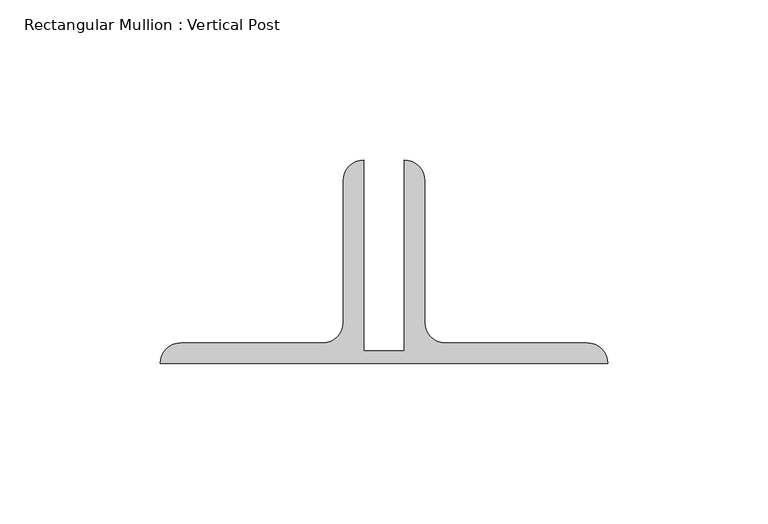
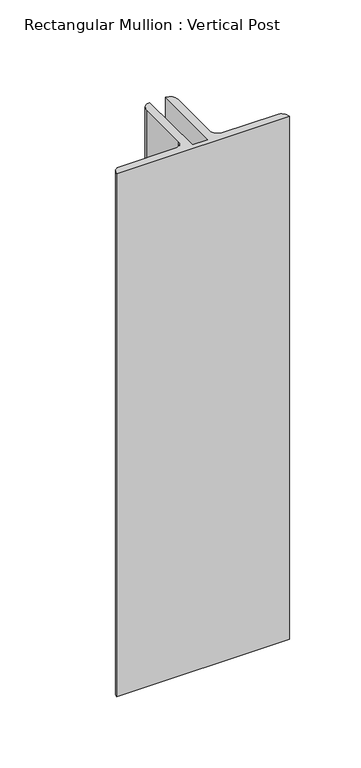
"""IFC4 building model written with IfcOpenShell, lengths in millimetres: member geometry, Rectangular Mullion : Vertical Post."""

import ifcopenshell
import ifcopenshell.guid

model = None  # the IFC model being written
_history = None  # IfcOwnerHistory: only IFC2X3 demands one
_inside = {}  # id of a spatial element -> (the spatial element, [elements in it])
_under = {}  # id of a project, library or spatial element -> (it, [spatial elements below it])
_declared = {}  # id of a project -> (the project, [libraries it declares])
_typed = {}  # id of a type object -> (the type object, [elements of that type])
_made_of = {}  # id of a material, layer set ... -> (it, [elements and type objects made of it])


def new_model(schema):
    """Start an empty IFC model of exactly this schema.

    Asked for "IFC4X3", IfcOpenShell would pick the latest addendum, in which some entities
    have other attributes; the version numbers below select the first issue.
    IFC2X3 requires an IfcOwnerHistory on every rooted entity: one is made here for all.
    """
    global model, _history
    if schema == "IFC4X3":
        model = ifcopenshell.file(schema_version=(4, 3, 0, 0))
    else:
        model = ifcopenshell.file(schema=schema)
    _inside.clear()
    _under.clear()
    _declared.clear()
    _typed.clear()
    _made_of.clear()
    _history = None
    if model.schema == "IFC2X3":
        org = make("IfcOrganization", Name="unknown")
        user = make(
            "IfcPersonAndOrganization",
            ThePerson=make("IfcPerson", FamilyName="unknown"),
            TheOrganization=org,
        )
        app = make(
            "IfcApplication",
            ApplicationDeveloper=org,
            Version="unknown",
            ApplicationFullName="unknown",
            ApplicationIdentifier="unknown",
        )
        _history = make(
            "IfcOwnerHistory",
            OwningUser=user,
            OwningApplication=app,
            ChangeAction="ADDED",
            CreationDate=0,
        )
    return model


def make(cls, **values):
    """One entity of the class cls with the attributes given. An attribute that is None is left unset."""
    return model.create_entity(
        cls, **{name: value for name, value in values.items() if value is not None}
    )


def rooted(cls, **values):
    """An entity with a GlobalId (a new one), such as an element, a storey or a relation."""
    return make(cls, GlobalId=ifcopenshell.guid.new(), OwnerHistory=_history, **values)


def si_unit(unit_type, name, prefix=None):
    """IfcSIUnit, for example si_unit("LENGTHUNIT", "METRE", prefix="MILLI")."""
    return make("IfcSIUnit", UnitType=unit_type, Prefix=prefix, Name=name)


def assignment(units):
    """IfcUnitAssignment: the units of a project."""
    return None if units is None else make("IfcUnitAssignment", Units=units)


def point(xyz):
    """IfcCartesianPoint."""
    return None if xyz is None else make("IfcCartesianPoint", Coordinates=xyz)


def direction(xyz):
    """IfcDirection."""
    return None if xyz is None else make("IfcDirection", DirectionRatios=xyz)


def frame(location, z_axis=None, x_axis=None):
    """IfcAxis2Placement3D, a coordinate frame: its origin and axes. An axis left out is left unset."""
    return make(
        "IfcAxis2Placement3D",
        Location=point(location),
        Axis=direction(z_axis),
        RefDirection=direction(x_axis),
    )


def frame_2d(location, x_axis=None):
    """IfcAxis2Placement2D, a coordinate frame in the plane: its origin and x axis."""
    return make(
        "IfcAxis2Placement2D", Location=point(location), RefDirection=direction(x_axis)
    )


def origin():
    """The frame at (0, 0, 0) with its axes left unset."""
    return frame((0.0, 0.0, 0.0))


def place(relative_to, where):
    """IfcLocalPlacement: puts the frame where relative to a parent placement (None: the world)."""
    return make(
        "IfcLocalPlacement", PlacementRelTo=relative_to, RelativePlacement=where
    )


def context(
    kind, dimensions, precision=None, world=None, true_north=None, identifier=None
):
    """IfcGeometricRepresentationContext, for example the 3D "Model" context."""
    return make(
        "IfcGeometricRepresentationContext",
        ContextIdentifier=identifier,
        ContextType=kind,
        CoordinateSpaceDimension=dimensions,
        Precision=precision,
        WorldCoordinateSystem=world,
        TrueNorth=true_north,
    )


def project(units=None, contexts=None):
    """IfcProject with its units and contexts."""
    return rooted(
        "IfcProject",
        Name="project",
        RepresentationContexts=contexts,
        UnitsInContext=assignment(units),
    )


def spatial(cls, under=None, at=None, **own):
    """A site, building, storey or space (cls), placed at a placement, below another one or the project."""
    s = rooted(cls, ObjectPlacement=at, **own)
    if under is not None:
        _under.setdefault(under.id(), (under, []))[1].append(s)
    return s


def polyline(points):
    """IfcPolyline through the points."""
    return make("IfcPolyline", Points=[point(p) for p in points])


def circle_curve(where, radius):
    """IfcCircle in the frame where."""
    return make("IfcCircle", Position=where, Radius=radius)


def trimmed(basis, trim1, trim2, sense, master):
    """IfcTrimmedCurve: the piece of a basis curve between two trims."""
    return make(
        "IfcTrimmedCurve",
        BasisCurve=basis,
        Trim1=trim1,
        Trim2=trim2,
        SenseAgreement=sense,
        MasterRepresentation=master,
    )


def segment(curve, same_sense, transition):
    """IfcCompositeCurveSegment."""
    return make(
        "IfcCompositeCurveSegment",
        Transition=transition,
        SameSense=same_sense,
        ParentCurve=curve,
    )


def composite_curve(segments, self_intersect=None):
    """IfcCompositeCurve: segments joined end to end."""
    return make("IfcCompositeCurve", Segments=segments, SelfIntersect=self_intersect)


def outline(outer, holes=None, kind="AREA"):
    """IfcArbitraryClosedProfileDef: a profile drawn as a closed curve; with holes, ...WithVoids."""
    if holes is None:
        return make("IfcArbitraryClosedProfileDef", ProfileType=kind, OuterCurve=outer)
    return make(
        "IfcArbitraryProfileDefWithVoids",
        ProfileType=kind,
        OuterCurve=outer,
        InnerCurves=holes,
    )


def extrude(swept, where, along, depth):
    """IfcExtrudedAreaSolid: the profile swept, set in the frame where, extruded along a direction by depth."""
    return make(
        "IfcExtrudedAreaSolid",
        SweptArea=swept,
        Position=where,
        ExtrudedDirection=direction(along),
        Depth=depth,
    )


def shape(context_of_items, identifier, shape_type, items):
    """IfcShapeRepresentation: the items that make up one representation, for example the "Body"."""
    return make(
        "IfcShapeRepresentation",
        ContextOfItems=context_of_items,
        RepresentationIdentifier=identifier,
        RepresentationType=shape_type,
        Items=items,
    )


def source(mapping_origin, context_of_items, identifier, shape_type, items):
    """IfcRepresentationMap: a shape defined once, which mapped items show again and again."""
    return make(
        "IfcRepresentationMap",
        MappingOrigin=mapping_origin,
        MappedRepresentation=shape(context_of_items, identifier, shape_type, items),
    )


def transform(
    local_origin,
    x_axis=None,
    y_axis=None,
    z_axis=None,
    scale=None,
    scale2=None,
    scale3=None,
    uniform=True,
):
    """IfcCartesianTransformationOperator3D, or its non-uniform kind. x_axis, y_axis, z_axis: its Axis1, 2, 3."""
    if uniform:
        return make(
            "IfcCartesianTransformationOperator3D",
            Axis1=direction(x_axis),
            Axis2=direction(y_axis),
            LocalOrigin=point(local_origin),
            Scale=scale,
            Axis3=direction(z_axis),
        )
    return make(
        "IfcCartesianTransformationOperator3DnonUniform",
        Axis1=direction(x_axis),
        Axis2=direction(y_axis),
        LocalOrigin=point(local_origin),
        Scale=scale,
        Axis3=direction(z_axis),
        Scale2=scale2,
        Scale3=scale3,
    )


def mapped(mapping_source, mapping_target):
    """IfcMappedItem: shows the shape of a source again, moved by a transform."""
    return make(
        "IfcMappedItem", MappingSource=mapping_source, MappingTarget=mapping_target
    )


def made_of(thing, what):
    """Note that an element or type object is made of a material, layer set ...; save() writes the relation."""
    if what is not None:
        _made_of.setdefault(what.id(), (what, []))[1].append(thing)
    return thing


def element(
    cls,
    number,
    at=None,
    inside=None,
    cuts=None,
    type_object=None,
    material=None,
    context=None,
    identifier="Body",
    shape_type=None,
    held_by="IfcProductDefinitionShape",
    body=None,
    shapes=None,
    **own,
):
    """One element of the class cls, such as IfcWall. Its Tag is "e" and its number.

    at: its placement. inside: the storey or other place that contains it. cuts: it is an
    opening in that element (IfcRelVoidsElement). A single representation is given by context,
    identifier, shape_type and body (its items); several are given by shapes. held_by: the class
    of the entity that holds the representations. save() writes the other relations.
    """
    e = rooted(cls, Tag="e%d" % number, ObjectPlacement=at, **own)
    if body is not None:
        shapes = [shape(context, identifier, shape_type, body)]
    if shapes is not None:
        e.Representation = make(held_by, Representations=shapes)
    if inside is not None:
        _inside.setdefault(inside.id(), (inside, []))[1].append(e)
    if cuts is not None:
        rooted(
            "IfcRelVoidsElement", RelatingBuildingElement=cuts, RelatedOpeningElement=e
        )
    if type_object is not None:
        _typed.setdefault(type_object.id(), (type_object, []))[1].append(e)
    return made_of(e, material)


def aggregate(whole, parts):
    """IfcRelAggregates: a whole, such as a stair, and the parts it consists of."""
    return rooted("IfcRelAggregates", RelatingObject=whole, RelatedObjects=parts)


def save(model, path):
    """Write the relations noted so far, then the file.

    IfcRelAggregates (storeys below a building ...), IfcRelContainedInSpatialStructure (elements
    in a storey), IfcRelDefinesByType, IfcRelAssociatesMaterial and IfcRelDeclares: one each for
    every whole, place, type object, material and project.
    """
    for whole, parts in _under.values():
        aggregate(whole, parts)
    for where, things in _inside.values():
        rooted(
            "IfcRelContainedInSpatialStructure",
            RelatedElements=things,
            RelatingStructure=where,
        )
    for kind, things in _typed.values():
        rooted("IfcRelDefinesByType", RelatedObjects=things, RelatingType=kind)
    for what, things in _made_of.values():
        rooted("IfcRelAssociatesMaterial", RelatedObjects=things, RelatingMaterial=what)
    for by, libraries in _declared.values():
        rooted("IfcRelDeclares", RelatingContext=by, RelatedDefinitions=libraries)
    model.write(path)


def rectangular_mullion_vertical_post_42193f95(model_context):
    return source(origin(), model_context, "Body", "SweptSolid", [
        extrude(outline(composite_curve([segment(polyline([(-76.2, 22.9145205), (-63.5, 22.9145205), (-63.5, 82.55)]), True, "CONTINUOUS"), segment(trimmed(circle_curve(frame_2d((-63.5, 76.2)), 6.35), [point((-63.5, 82.55))], [point((-57.15, 76.2))], False, "CARTESIAN"), True, "CONTINUOUS"), segment(polyline([(-57.15, 76.2), (-57.15, 31.75)]), True, "CONTINUOUS"), segment(trimmed(circle_curve(frame_2d((-50.8, 31.75)), 6.35), [point((-57.15, 31.75))], [point((-50.8, 25.4))], True, "CARTESIAN"), True, "CONTINUOUS"), segment(polyline([(-50.8, 25.4), (-6.35, 25.4)]), True, "CONTINUOUS"), segment(trimmed(circle_curve(frame_2d((-6.35, 19.05)), 6.35), [point((-6.35, 25.4))], [point((0.0, 19.05))], False, "CARTESIAN"), True, "CONTINUOUS"), segment(polyline([(0.0, 19.05), (-139.7, 19.05)]), True, "CONTINUOUS"), segment(trimmed(circle_curve(frame_2d((-133.35, 19.05)), 6.35), [point((-139.7, 19.05))], [point((-133.35, 25.4))], False, "CARTESIAN"), True, "CONTINUOUS"), segment(polyline([(-133.35, 25.4), (-88.9, 25.4)]), True, "CONTINUOUS"), segment(trimmed(circle_curve(frame_2d((-88.9, 31.75)), 6.35), [point((-88.9, 25.4))], [point((-82.55, 31.75))], True, "CARTESIAN"), True, "CONTINUOUS"), segment(polyline([(-82.55, 31.75), (-82.55, 76.2)]), True, "CONTINUOUS"), segment(trimmed(circle_curve(frame_2d((-76.2, 76.2)), 6.35), [point((-82.55, 76.2))], [point((-76.2, 82.55))], False, "CARTESIAN"), True, "CONTINUOUS"), segment(polyline([(-76.2, 82.55), (-76.2, 22.9145205)]), True, "CONTINUOUS")], self_intersect=False)), frame((0.0, 0.0, -446.7663052), z_axis=(0.0, 0.0, 1.0), x_axis=(1.0, 0.0, 0.0)), (0.0, 0.0, 1.0), 446.7663052),
    ])


if __name__ == "__main__":
    model = new_model("IFC4")
    model_context = context("Model", 3, world=origin())
    ifc_project = project(units=[si_unit("LENGTHUNIT", "METRE", prefix="MILLI")], contexts=[model_context])
    site = spatial("IfcSite", under=ifc_project)
    building = spatial("IfcBuilding", under=site)
    placement = place(None, origin())
    rectangular_mullion_vertical_post_shape = rectangular_mullion_vertical_post_42193f95(model_context)
    element("IfcMember", 1, ObjectType="Rectangular Mullion : Vertical Post", at=placement, inside=building, context=model_context, shape_type="MappedRepresentation", body=[
        mapped(rectangular_mullion_vertical_post_shape, transform((0.0, 0.0, 0.0), x_axis=(1.0, 0.0, 0.0), y_axis=(0.0, 1.0, 0.0), z_axis=(0.0, 0.0, 1.0))),
    ])
    save(model, "model.ifc")

# Revit data of these elements
# Type "Rectangular Mullion : Vertical Post"
#   built-in parameter 1007351 = -0.0625 (stored number, unit not read)
#   built-in parameter 1007322 = 0.0126789 (stored number, unit not read)
#   built-in parameter 1007321 = 0.229167 (stored number, unit not read)
#   built-in parameter 1007320 = 0.229167 (stored number, unit not read)
# Element 1 (IfcMember, "Rectangular Mullion : Vertical Post")
#   Materials on its faces: "GATE POST: (2) BACK/BACK GALVANIZED ANGLES"
# Materials
#   "GATE POST: (2) BACK/BACK GALVANIZED ANGLES": class "Unassigned", colour RGB 211 211 211, transparency 0, Cost = 0
